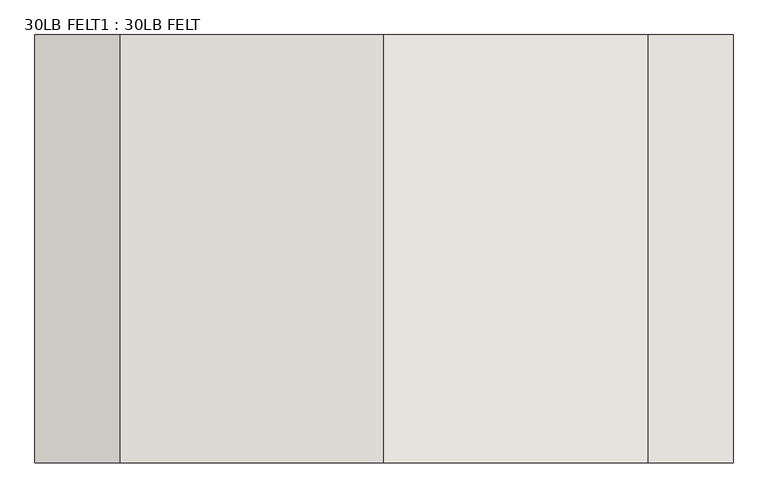
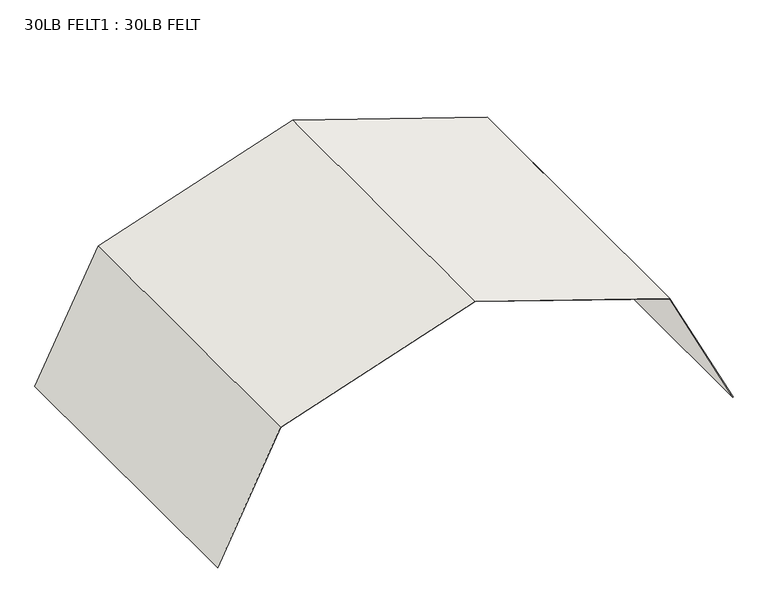
"""IFC4 building model written with IfcOpenShell, lengths in millimetres: wall geometry, 30LB FELT1 : 30LB FELT."""

from ifc_helpers import new_model, si_unit, frame, origin, place, context, project, spatial, polyline, outline, extrude, source, transform, mapped, element, save


def wall_30lb_felt1_30lb_felt_e6985e1f(model_context):
    return source(origin(), model_context, "Body", "SweptSolid", [
        extrude(outline(polyline([(4135.7392702, 23778.3109518), (5279.4659735, 23206.4476002), (5869.2725154, 21444.7370052), (5279.4659735, 19683.0264102), (4135.8949093, 19111.2408782), (4135.1849577, 19112.6607813), (5278.1689698, 19684.1527874), (5867.5984097, 21444.7370052), (5278.1689698, 23205.321223), (4135.0293186, 23776.8910486), (4135.7392702, 23778.3109518)])), frame((0.0, -3415.0384634, 0.0), z_axis=(0.0, 1.0, 0.0), x_axis=(0.0, 0.0, 1.0)), (0.0, 0.0, 1.0), 2862.7206389),
    ])


if __name__ == "__main__":
    model = new_model("IFC4")
    model_context = context("Model", 3, world=origin())
    ifc_project = project(units=[si_unit("LENGTHUNIT", "METRE", prefix="MILLI")], contexts=[model_context])
    site = spatial("IfcSite", under=ifc_project)
    building = spatial("IfcBuilding", under=site)
    placement = place(None, origin())
    wall_30lb_felt1_30lb_felt_shape = wall_30lb_felt1_30lb_felt_e6985e1f(model_context)
    element("IfcWall", 1, ObjectType="30LB FELT1 : 30LB FELT", at=placement, inside=building, context=model_context, shape_type="MappedRepresentation", body=[
        mapped(wall_30lb_felt1_30lb_felt_shape, transform((0.0, 0.0, 0.0), x_axis=(1.0, 0.0, 0.0), y_axis=(0.0, 1.0, 0.0), z_axis=(0.0, 0.0, 1.0))),
    ])
    save(model, "model.ifc")

# Revit data of these elements
# Element 1 (IfcWall, "30LB FELT1 : 30LB FELT")
#   Materials on its faces: "30LB FELT"
# Materials
#   "30LB FELT": class "Generic", colour RGB 66 158 52, transparency 0, Cost = 0
